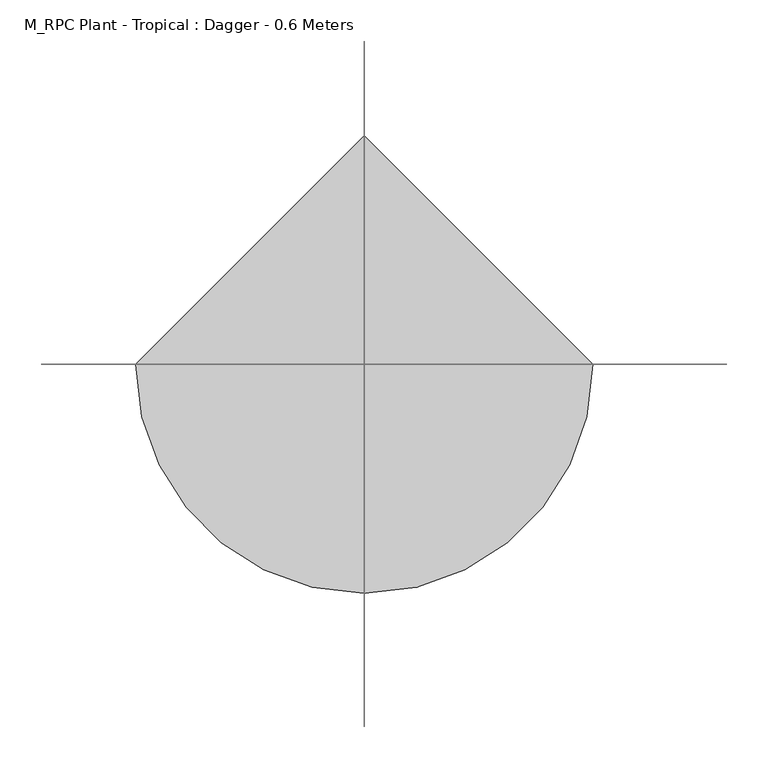
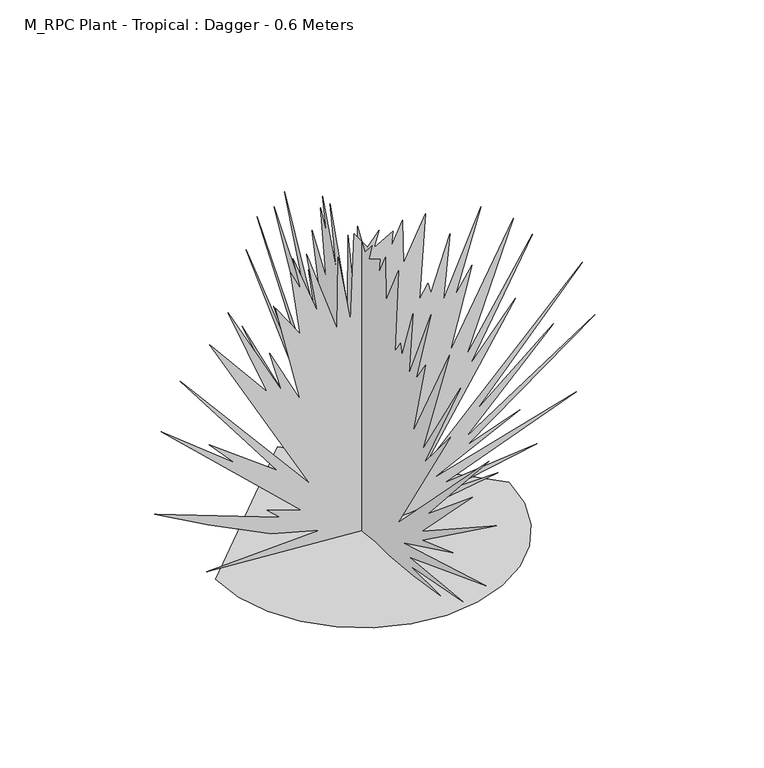
"""IFC4 building model written with IfcOpenShell, lengths in millimetres: geographic element geometry, M_RPC Plant - Tropical : Dagger - 0.6 Meters."""

import ifcopenshell
import ifcopenshell.guid

model = None  # the IFC model being written
_history = None  # IfcOwnerHistory: only IFC2X3 demands one
_inside = {}  # id of a spatial element -> (the spatial element, [elements in it])
_under = {}  # id of a project, library or spatial element -> (it, [spatial elements below it])
_declared = {}  # id of a project -> (the project, [libraries it declares])
_typed = {}  # id of a type object -> (the type object, [elements of that type])
_made_of = {}  # id of a material, layer set ... -> (it, [elements and type objects made of it])


def new_model(schema):
    """Start an empty IFC model of exactly this schema.

    Asked for "IFC4X3", IfcOpenShell would pick the latest addendum, in which some entities
    have other attributes; the version numbers below select the first issue.
    IFC2X3 requires an IfcOwnerHistory on every rooted entity: one is made here for all.
    """
    global model, _history
    if schema == "IFC4X3":
        model = ifcopenshell.file(schema_version=(4, 3, 0, 0))
    else:
        model = ifcopenshell.file(schema=schema)
    _inside.clear()
    _under.clear()
    _declared.clear()
    _typed.clear()
    _made_of.clear()
    _history = None
    if model.schema == "IFC2X3":
        org = make("IfcOrganization", Name="unknown")
        user = make(
            "IfcPersonAndOrganization",
            ThePerson=make("IfcPerson", FamilyName="unknown"),
            TheOrganization=org,
        )
        app = make(
            "IfcApplication",
            ApplicationDeveloper=org,
            Version="unknown",
            ApplicationFullName="unknown",
            ApplicationIdentifier="unknown",
        )
        _history = make(
            "IfcOwnerHistory",
            OwningUser=user,
            OwningApplication=app,
            ChangeAction="ADDED",
            CreationDate=0,
        )
    return model


def make(cls, **values):
    """One entity of the class cls with the attributes given. An attribute that is None is left unset."""
    return model.create_entity(
        cls, **{name: value for name, value in values.items() if value is not None}
    )


def rooted(cls, **values):
    """An entity with a GlobalId (a new one), such as an element, a storey or a relation."""
    return make(cls, GlobalId=ifcopenshell.guid.new(), OwnerHistory=_history, **values)


def si_unit(unit_type, name, prefix=None):
    """IfcSIUnit, for example si_unit("LENGTHUNIT", "METRE", prefix="MILLI")."""
    return make("IfcSIUnit", UnitType=unit_type, Prefix=prefix, Name=name)


def assignment(units):
    """IfcUnitAssignment: the units of a project."""
    return None if units is None else make("IfcUnitAssignment", Units=units)


def point(xyz):
    """IfcCartesianPoint."""
    return None if xyz is None else make("IfcCartesianPoint", Coordinates=xyz)


def direction(xyz):
    """IfcDirection."""
    return None if xyz is None else make("IfcDirection", DirectionRatios=xyz)


def frame(location, z_axis=None, x_axis=None):
    """IfcAxis2Placement3D, a coordinate frame: its origin and axes. An axis left out is left unset."""
    return make(
        "IfcAxis2Placement3D",
        Location=point(location),
        Axis=direction(z_axis),
        RefDirection=direction(x_axis),
    )


def origin():
    """The frame at (0, 0, 0) with its axes left unset."""
    return frame((0.0, 0.0, 0.0))


def place(relative_to, where):
    """IfcLocalPlacement: puts the frame where relative to a parent placement (None: the world)."""
    return make(
        "IfcLocalPlacement", PlacementRelTo=relative_to, RelativePlacement=where
    )


def context(
    kind, dimensions, precision=None, world=None, true_north=None, identifier=None
):
    """IfcGeometricRepresentationContext, for example the 3D "Model" context."""
    return make(
        "IfcGeometricRepresentationContext",
        ContextIdentifier=identifier,
        ContextType=kind,
        CoordinateSpaceDimension=dimensions,
        Precision=precision,
        WorldCoordinateSystem=world,
        TrueNorth=true_north,
    )


def project(units=None, contexts=None):
    """IfcProject with its units and contexts."""
    return rooted(
        "IfcProject",
        Name="project",
        RepresentationContexts=contexts,
        UnitsInContext=assignment(units),
    )


def spatial(cls, under=None, at=None, **own):
    """A site, building, storey or space (cls), placed at a placement, below another one or the project."""
    s = rooted(cls, ObjectPlacement=at, **own)
    if under is not None:
        _under.setdefault(under.id(), (under, []))[1].append(s)
    return s


def point_list(points):
    """IfcCartesianPointList2D or 3D."""
    cls = (
        "IfcCartesianPointList2D" if len(points[0]) == 2 else "IfcCartesianPointList3D"
    )
    return make(cls, CoordList=points)


def triangles(points, corners, closed=None, point_numbers=None):
    """IfcTriangulatedFaceSet: each triangle names its three corners, points numbered from 1."""
    return make(
        "IfcTriangulatedFaceSet",
        Coordinates=point_list(points),
        Closed=closed,
        CoordIndex=corners,
        PnIndex=point_numbers,
    )


def shape(context_of_items, identifier, shape_type, items):
    """IfcShapeRepresentation: the items that make up one representation, for example the "Body"."""
    return make(
        "IfcShapeRepresentation",
        ContextOfItems=context_of_items,
        RepresentationIdentifier=identifier,
        RepresentationType=shape_type,
        Items=items,
    )


def source(mapping_origin, context_of_items, identifier, shape_type, items):
    """IfcRepresentationMap: a shape defined once, which mapped items show again and again."""
    return make(
        "IfcRepresentationMap",
        MappingOrigin=mapping_origin,
        MappedRepresentation=shape(context_of_items, identifier, shape_type, items),
    )


def transform(
    local_origin,
    x_axis=None,
    y_axis=None,
    z_axis=None,
    scale=None,
    scale2=None,
    scale3=None,
    uniform=True,
):
    """IfcCartesianTransformationOperator3D, or its non-uniform kind. x_axis, y_axis, z_axis: its Axis1, 2, 3."""
    if uniform:
        return make(
            "IfcCartesianTransformationOperator3D",
            Axis1=direction(x_axis),
            Axis2=direction(y_axis),
            LocalOrigin=point(local_origin),
            Scale=scale,
            Axis3=direction(z_axis),
        )
    return make(
        "IfcCartesianTransformationOperator3DnonUniform",
        Axis1=direction(x_axis),
        Axis2=direction(y_axis),
        LocalOrigin=point(local_origin),
        Scale=scale,
        Axis3=direction(z_axis),
        Scale2=scale2,
        Scale3=scale3,
    )


def mapped(mapping_source, mapping_target):
    """IfcMappedItem: shows the shape of a source again, moved by a transform."""
    return make(
        "IfcMappedItem", MappingSource=mapping_source, MappingTarget=mapping_target
    )


def made_of(thing, what):
    """Note that an element or type object is made of a material, layer set ...; save() writes the relation."""
    if what is not None:
        _made_of.setdefault(what.id(), (what, []))[1].append(thing)
    return thing


def element(
    cls,
    number,
    at=None,
    inside=None,
    cuts=None,
    type_object=None,
    material=None,
    context=None,
    identifier="Body",
    shape_type=None,
    held_by="IfcProductDefinitionShape",
    body=None,
    shapes=None,
    **own,
):
    """One element of the class cls, such as IfcWall. Its Tag is "e" and its number.

    at: its placement. inside: the storey or other place that contains it. cuts: it is an
    opening in that element (IfcRelVoidsElement). A single representation is given by context,
    identifier, shape_type and body (its items); several are given by shapes. held_by: the class
    of the entity that holds the representations. save() writes the other relations.
    """
    e = rooted(cls, Tag="e%d" % number, ObjectPlacement=at, **own)
    if body is not None:
        shapes = [shape(context, identifier, shape_type, body)]
    if shapes is not None:
        e.Representation = make(held_by, Representations=shapes)
    if inside is not None:
        _inside.setdefault(inside.id(), (inside, []))[1].append(e)
    if cuts is not None:
        rooted(
            "IfcRelVoidsElement", RelatingBuildingElement=cuts, RelatedOpeningElement=e
        )
    if type_object is not None:
        _typed.setdefault(type_object.id(), (type_object, []))[1].append(e)
    return made_of(e, material)


def aggregate(whole, parts):
    """IfcRelAggregates: a whole, such as a stair, and the parts it consists of."""
    return rooted("IfcRelAggregates", RelatingObject=whole, RelatedObjects=parts)


def save(model, path):
    """Write the relations noted so far, then the file.

    IfcRelAggregates (storeys below a building ...), IfcRelContainedInSpatialStructure (elements
    in a storey), IfcRelDefinesByType, IfcRelAssociatesMaterial and IfcRelDeclares: one each for
    every whole, place, type object, material and project.
    """
    for whole, parts in _under.values():
        aggregate(whole, parts)
    for where, things in _inside.values():
        rooted(
            "IfcRelContainedInSpatialStructure",
            RelatedElements=things,
            RelatingStructure=where,
        )
    for kind, things in _typed.values():
        rooted("IfcRelDefinesByType", RelatedObjects=things, RelatingType=kind)
    for what, things in _made_of.values():
        rooted("IfcRelAssociatesMaterial", RelatedObjects=things, RelatingMaterial=what)
    for by, libraries in _declared.values():
        rooted("IfcRelDeclares", RelatingContext=by, RelatedDefinitions=libraries)
    model.write(path)


def m_rpc_plant_tropical_dagger_0_6_meters_3415abb8(model_context):
    return source(origin(), model_context, "Body", "Tessellation", [
        triangles([(0.1799897, -5.7252047, 0.0), (0.1800089, 294.2752427, 20.8333418), (0.1799966, 80.3860635, 29.1667744), (0.1800035, 172.052634, 54.1667927), (0.1800144, 292.8852294, 115.2778473), (0.1800237, 392.885321, 170.8333952), (0.1800042, 155.3861186, 81.9445621), (0.180007, 180.386137, 104.166834), (0.1800018, 115.1083446, 81.9445621), (0.1800325, 380.3853209, 331.9452544), (0.1800176, 241.4971961, 220.8334319), (0.1800237, 290.1077282, 273.610225), (0.1800103, 160.9416298, 177.7779023), (0.1800356, 344.2752794, 419.4453278), (0.1800038, 99.8305798, 130.555603), (0.1800355, 288.7202402, 473.6103719), (0.1800212, 180.386137, 341.6677714), (0.1800365, 253.9977048, 525.00044), (0.1800191, 152.6083812, 334.7227738), (0.1800253, 174.8306439, 416.6678447), (0.1800152, 117.8860911, 304.167753), (0.1800298, 163.7193854, 502.7779229), (0.1800231, 117.8860911, 436.1103353), (0.1800318, 135.9416114, 563.8904717), (0.1800283, 116.4970952, 525.00044), (0.180033, 130.3861093, 590.2779599), (0.180023, 84.5525697, 468.0553694), (0.1800315, 105.3860819, 590.2779599), (0.1800179, 47.0527875, 420.8328521), (0.1800264, 45.663787, 563.8904717), (0.1800169, 22.052617, 427.7778497), (0.1800267, 15.1081371, 600.0004769), (0.1800231, -9.8918086, 563.8904717), (0.1800233, -32.1140259, 590.2779599), (0.180022, -22.3918427, 558.3329621), (0.1800211, -58.503047, 579.1679549), (0.1800196, -55.7252959, 551.3904353), (0.1800209, -76.5585628, 594.4454744), (0.1800157, -77.9475587, 508.3329254), (0.1800183, -119.6140924, 593.0554793), (0.1800089, -108.5030882, 425.0003303), (0.1800095, -125.1698489, 451.3903619), (0.180008, -130.7253601, 430.5553328), (0.1800121, -166.8363826, 536.110445), (0.1800052, -154.3363825, 408.3328156), (0.1800106, -225.1696861, 569.4454742), (0.180004, -176.5586453, 411.1103351), (0.180005, -208.5031707, 458.3328524), (0.179998, -166.8363826, 300.0002385), (0.1800043, -286.2802365, 525.00044), (0.1799951, -197.3919122, 281.9452359), (0.1799995, -322.3927488, 480.5554058), (0.1799934, -204.3364192, 261.1102067), (0.1799944, -290.4477329, 363.8902885), (0.1799882, -118.2253418, 87.5000733), (0.1799886, -416.8378198, 391.6678082), (0.1799871, -215.4476778, 165.277884), (0.1799856, -362.6703049, 287.5002384), (0.1799854, -196.0031525, 118.0555938), (0.1799804, -440.4478612, 277.7777214), (0.1799843, -198.7809081, 101.3890784), (0.1799804, -298.7802366, 137.5001101), (0.1799855, -134.8918572, 58.333299), (0.179974, -405.725344, 136.1111142), (0.1799833, -155.7253784, 41.6667836), (0.1799738, -330.7252707, 58.333299), (0.1799822, -157.11412, 25.0000206), (0.1799763, -257.1152108, 26.3890211), (0.1799808, -168.2253785, 12.5000103), (0.1799851, -87.669567, 4.1666533), (0.1799877, -43.2252867, 4.1666533), (-277.616067, 0.0, 0.0922626), (-270.2710575, -63.6563025, 0.0922626), (-249.3550376, -122.1146029, 0.0922626), (-216.5405072, -173.699899, 0.0922626), (-173.5032359, -216.7371703, 0.0922626), (-121.9179307, -249.5517008, 0.0922626), (-63.4596303, -270.4677206, 0.0922626), (0.1966832, -277.8127301, 0.0922626), (63.8529748, -270.4677206, 0.0922626), (122.3112752, -249.5517008, 0.0922626), (173.8965621, -216.7371703, 0.0922626), (216.9338335, -173.699899, 0.0922626), (249.7483639, -122.1146029, 0.0922626), (270.6643837, -63.6563025, 0.0922626), (278.0093933, 2.43e-05, 0.0922626), (0.1966346, 277.8127301, 0.0922626), (5.9218758, 0.016681, 0.0), (-294.0785796, 0.0166798, 20.8333418), (-80.1893913, 0.0166793, 29.1667744), (-171.8562252, 0.0166778, 54.1667927), (-292.6885663, 0.0166741, 115.2778473), (-392.6886397, 0.0166708, 170.8333952), (-155.1894555, 0.0166761, 81.9445621), (-180.1894738, 0.0166748, 104.166834), (-114.9116723, 0.0166761, 81.9445621), (-380.1886396, 0.0166612, 331.9452544), (-241.3005329, 0.0166679, 220.8334319), (-289.9110651, 0.0166647, 273.610225), (-160.7449667, 0.0166704, 177.7779023), (-344.0785981, 0.016656, 419.4453278), (-99.6339076, 0.0166732, 130.555603), (-288.5235771, 0.0166528, 473.6103719), (-180.1894738, 0.0166607, 341.6677714), (-253.8010417, 0.0166497, 525.00044), (-152.411718, 0.0166611, 334.7227738), (-174.6339808, 0.0166562, 416.6678447), (-117.6894188, 0.0166629, 304.167753), (-163.5227222, 0.016651, 502.7779229), (-117.6894188, 0.016655, 436.1103353), (-135.7449392, 0.0166474, 563.8904717), (-116.300423, 0.0166497, 525.00044), (-130.1894371, 0.0166458, 590.2779599), (-84.3558975, 0.0166531, 468.0553694), (-105.1894097, 0.0166458, 590.2779599), (-46.8561152, 0.0166559, 420.8328521), (-45.4671148, 0.0166474, 563.8904717), (-21.855947, 0.0166555, 427.7778497), (-14.911491, 0.0166453, 600.0004769), (10.0885046, 0.0166474, 563.8904717), (32.3106959, 0.0166458, 590.2779599), (22.5885127, 0.0166477, 558.3329621), (58.6997192, 0.0166465, 579.1679549), (55.9219681, 0.0166481, 551.3904353), (76.755235, 0.0166456, 594.4454744), (78.1442309, 0.0166507, 508.3329254), (119.8107646, 0.0166457, 593.0554793), (108.6997604, 0.0166557, 425.0003303), (125.3665211, 0.0166541, 451.3903619), (130.9220323, 0.0166553, 430.5553328), (167.0330458, 0.0166491, 536.110445), (154.5330457, 0.0166567, 408.3328156), (225.3663493, 0.0166471, 569.4454742), (176.7553084, 0.0166565, 411.1103351), (208.6998339, 0.0166537, 458.3328524), (167.0330458, 0.0166631, 300.0002385), (286.4768997, 0.0166497, 525.00044), (197.5885753, 0.0166642, 281.9452359), (322.5894301, 0.0166524, 480.5554058), (204.5330824, 0.0166655, 261.1102067), (290.644396, 0.0166593, 363.8902885), (118.422014, 0.0166758, 87.5000733), (417.0345011, 0.0166577, 391.6678082), (215.6443409, 0.0166712, 165.277884), (362.8669862, 0.0166639, 287.5002384), (196.1998156, 0.016674, 118.0555938), (440.6445425, 0.0166645, 277.7777214), (198.9775712, 0.016675, 101.3890784), (298.9768998, 0.0166728, 137.5001101), (135.0885294, 0.0166776, 58.333299), (405.9220253, 0.0166729, 136.1111142), (155.9220416, 0.0166785, 41.6667836), (330.9219521, 0.0166776, 58.333299), (157.3107831, 0.0166795, 25.0000206), (257.3118739, 0.0166795, 26.3890211), (168.4220417, 0.0166803, 12.5000103), (87.8662392, 0.0166808, 4.1666533), (43.4219589, 0.0166808, 4.1666533)], [[68, 67, 69], [69, 67, 70], [64, 63, 65], [62, 61, 63], [58, 57, 59], [56, 55, 57], [57, 55, 59], [52, 51, 53], [50, 49, 51], [48, 47, 49], [46, 45, 47], [47, 45, 49], [40, 39, 41], [36, 35, 37], [34, 33, 35], [28, 27, 29], [26, 25, 27], [24, 23, 25], [22, 21, 23], [20, 19, 21], [16, 15, 17], [12, 11, 13], [10, 9, 11], [11, 9, 13], [8, 7, 9], [2, 1, 3], [66, 65, 67], [67, 65, 70], [65, 63, 70], [60, 59, 61], [61, 59, 63], [59, 55, 63], [63, 55, 70], [54, 53, 55], [53, 51, 55], [51, 49, 55], [49, 45, 55], [44, 43, 45], [45, 43, 55], [43, 42, 55], [42, 41, 55], [55, 41, 70], [41, 39, 70], [70, 39, 71], [39, 38, 71], [38, 37, 71], [37, 35, 71], [71, 35, 1], [35, 33, 1], [33, 32, 1], [18, 17, 19], [17, 15, 19], [19, 15, 21], [14, 13, 15], [13, 9, 15], [6, 5, 7], [5, 4, 7], [4, 3, 7], [7, 3, 9], [9, 3, 15], [21, 15, 23], [23, 15, 25], [25, 15, 27], [15, 3, 27], [27, 3, 29], [3, 1, 29], [29, 1, 30], [30, 1, 31], [1, 32, 31], [86, 87, 72], [85, 86, 72], [85, 72, 73], [84, 85, 73], [84, 73, 74], [84, 74, 75], [83, 84, 75], [82, 83, 75], [82, 75, 76], [82, 76, 77], [82, 77, 78], [82, 78, 79], [82, 79, 80], [82, 80, 81], [154, 155, 156], [154, 156, 157], [150, 151, 152], [148, 149, 150], [144, 145, 146], [142, 143, 144], [142, 144, 146], [138, 139, 140], [136, 137, 138], [134, 135, 136], [132, 133, 134], [132, 134, 136], [126, 127, 128], [122, 123, 124], [120, 121, 122], [114, 115, 116], [112, 113, 114], [110, 111, 112], [108, 109, 110], [106, 107, 108], [102, 103, 104], [98, 99, 100], [96, 97, 98], [96, 98, 100], [94, 95, 96], [88, 89, 90], [152, 153, 154], [152, 154, 157], [150, 152, 157], [146, 147, 148], [146, 148, 150], [142, 146, 150], [142, 150, 157], [140, 141, 142], [138, 140, 142], [136, 138, 142], [132, 136, 142], [130, 131, 132], [130, 132, 142], [129, 130, 142], [128, 129, 142], [128, 142, 157], [126, 128, 157], [126, 157, 158], [125, 126, 158], [124, 125, 158], [122, 124, 158], [122, 158, 88], [120, 122, 88], [119, 120, 88], [104, 105, 106], [102, 104, 106], [102, 106, 108], [100, 101, 102], [96, 100, 102], [92, 93, 94], [91, 92, 94], [90, 91, 94], [90, 94, 96], [90, 96, 102], [102, 108, 110], [102, 110, 112], [102, 112, 114], [90, 102, 114], [90, 114, 116], [88, 90, 116], [88, 116, 117], [88, 117, 118], [119, 88, 118]], closed=False),
    ])


if __name__ == "__main__":
    model = new_model("IFC4")
    model_context = context("Model", 3, world=origin())
    ifc_project = project(units=[si_unit("LENGTHUNIT", "METRE", prefix="MILLI")], contexts=[model_context])
    site = spatial("IfcSite", under=ifc_project)
    building = spatial("IfcBuilding", under=site)
    placement = place(None, origin())
    m_rpc_plant_tropical_dagger_0_6_meters_shape = m_rpc_plant_tropical_dagger_0_6_meters_3415abb8(model_context)
    element("IfcGeographicElement", 1, ObjectType="M_RPC Plant - Tropical : Dagger - 0.6 Meters", at=placement, inside=building, context=model_context, shape_type="MappedRepresentation", body=[
        mapped(m_rpc_plant_tropical_dagger_0_6_meters_shape, transform((0.0, 0.0, 0.0), x_axis=(1.0, 0.0, 0.0), y_axis=(0.0, 1.0, 0.0), z_axis=(0.0, 0.0, 1.0))),
    ])
    save(model, "model.ifc")

# Revit data of these elements
# Type "M_RPC Plant - Tropical : Dagger - 0.6 Meters"
#   built-in parameter 1005198 = "{2, 15},{39, RPC-16-G3A7-NEG0-UH6H-J000-ST1L-LVER-AU},{1, 0},{1, 0},{2, 35},{1, 8},{5, Color},{1, 0},{1, 0},{3, 0.8},{3, 0.8},{3, 0.8},{1, 8},{7, BBoxMin},{1, 0},{1, 0},{1, 0},{1, 0},{1, 0},{1, 8},{7, BBoxMax},{1, 0},{1, 0},{1, 0},{1, 0},{1, 0},{2, 11},{9, RPCTypeId},{1, 0},{1, 0},{39, RPC-16-G3A7-NEG0-UH6H-J000-ST1L-LVER-AU},{1, 6},{14, RPCPlantHeight},{1, 0},{1, 0},{6, 1.9685},{2, 11},{7, keyword},{1, 0},{1, 0},{55, :Geometry:RPC:Dagger:Yucca Recurvifolia:plant:tropical.},{2, 11},{8, category},{1, 0},{1, 0},{17, :Plants [General]},{2, 11},{12, LocalizedUID},{1, 0},{1, 0},{6, Dagger},{2, 14},{6, Height},{1, 0},{1, 0},{6, 1.9685},{1, 2},{16, Cast Reflections},{1, 0},{1, 0},{1, 0},{1, 2},{12, Cast Shadows},{1, 0},{1, 0},{1, 1},{1, 2},{9, Lock View},{1, 0},{1, 0},{1, 0},{1, 4},{5, ViewC},{1, 0},{1, 0},{1, 0},{2, 11},{20, AdvancedUIDefinition},{1, 0},{1, 0},{0, },{2, 11},{10, AssetLibID},{1, 0},{1, 0},{36, 4D3F6E72-3F99-4203-98E9-AF80B3C7A7A4},{2, 11},{10, BaseSchema},{1, 0},{1, 0},{9, RPCSchema},{2, 11},{12, ExchangeGUID},{1, 0},{1, 0},{0, },{1, 2},{6, Hidden},{1, 0},{1, 0},{1, 0},{1, 4},{11, RPCCategory},{1, 0},{1, 0},{1, 0},{2, 11},{8, RPCImage},{1, 0},{1, 0},{0, },{1, 4},{13, SchemaVersion},{1, 0},{1, 0},{1, 4},{2, 11},{12, UIDefinition},{1, 0},{1, 0},{0, },{2, 11},{6, UIName},{1, 0},{1, 0},{39, RPC-16-G3A7-NEG0-UH6H-J000-ST1L-LVER-AU},{2, 11},{11, VersionGUID},{1, 0},{1, 0},{9, RPCSchema},{2, 11},{9, assettype},{1, 0},{1, 0},{11, RPCGeometry},{2, 11},{11, description},{1, 0},{1, 0},{0, },{2, 11},{9, localname},{1, 0},{1, 0},{3, RPC},{2, 11},{9, localtype},{1, 0},{1, 0},{3, RPC},{1, 4},{8, revision},{1, 0},{1, 0},{1, 1},{2, 11},{9, thumbnail},{1, 0},{1, 0},{0, },{1, 4},{7, version},{1, 0},{1, 0},{1, 1},{1, 2},{20, RPC_Cast Reflections},{1, 0},{1, 0},{1, 1},{1, 2},{16, RPC_Cast Shadows},{1, 0},{1, 0},{1, 1},{1, 2},{13, RPC_Lock View},{1, 0},{1, 0},{1, 0},{1, 4},{9, RPC_ViewC},{1, 0},{1, 0},{1, 0},{21, assetlibrary_base.fbx},{1, 5},"
#   built-in parameter 1005195 = "RPC-16-G3A7-NEG0-UH6H-J000-ST1L-LVER-AU"
#   Type Comments = "Dagger"
#   Height = 0.6 m
#   Description = (empty or 0)
#   Default Elevation = 0
